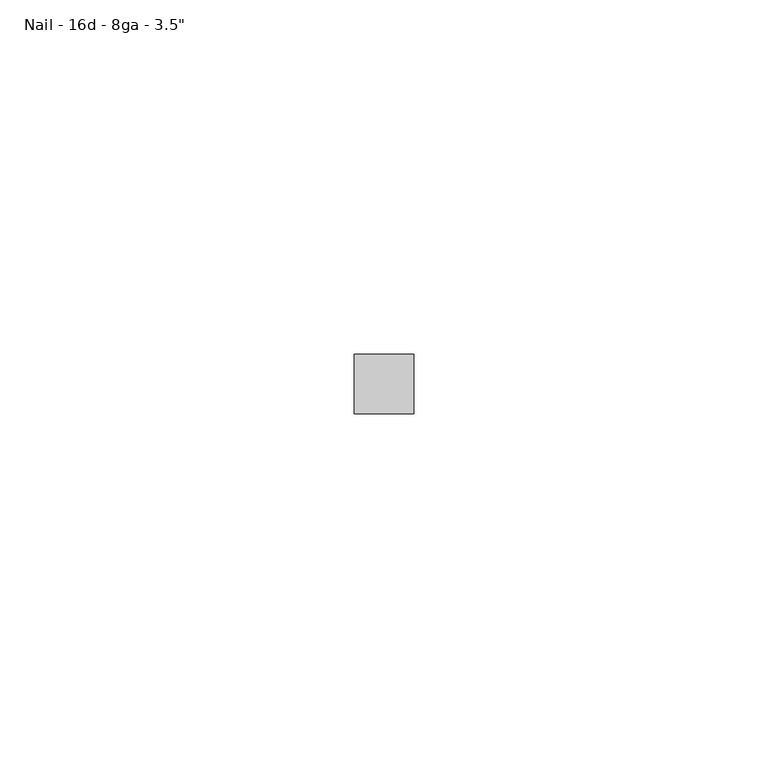
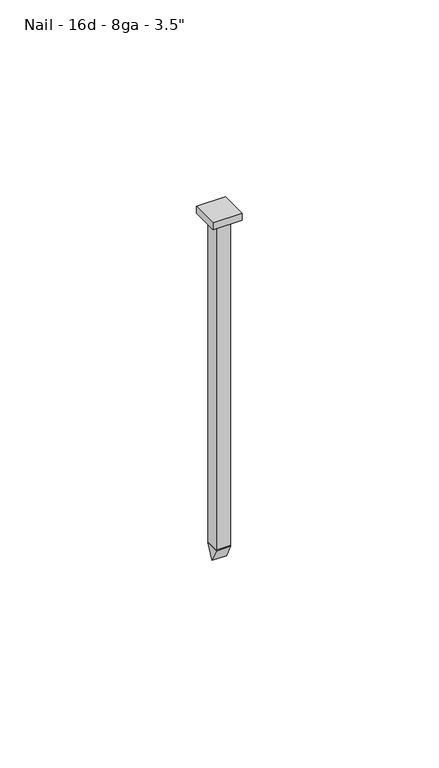
"""IFC4 building model written with IfcOpenShell, lengths in millimetres: fastener geometry."""

from ifc_helpers import new_model, si_unit, frame, origin, origin_with_axes, place, context, project, spatial, polyline, outline, extrude, source, transform, mapped, element, save


def fastener_034bf7df(model_context):
    return source(origin(), model_context, "Body", "SweptSolid", [
        extrude(outline(polyline([(0.0, -105.791), (-2.0955, -101.6), (2.0955, -101.6), (0.0, -105.791)])), frame((-2.0955, 0.0, 0.0), z_axis=(1.0, 0.0, 0.0), x_axis=(0.0, 1.0, 0.0)), (0.0, 0.0, 1.0), 4.191),
        extrude(outline(polyline([(-4.191, -4.191), (-4.191, 4.191), (4.191, 4.191), (4.191, -4.191), (-4.191, -4.191)])), origin_with_axes(), (0.0, 0.0, 1.0), 2.0955),
        extrude(outline(polyline([(-2.0955, 2.0955), (2.0955, 2.0955), (2.0955, -2.0955), (-2.0955, -2.0955), (-2.0955, 2.0955)])), frame((0.0, 0.0, -101.6), z_axis=(0.0, 0.0, 1.0), x_axis=(1.0, 0.0, 0.0)), (0.0, 0.0, 1.0), 101.6),
    ])


if __name__ == "__main__":
    model = new_model("IFC4")
    model_context = context("Model", 3, world=origin())
    ifc_project = project(units=[si_unit("LENGTHUNIT", "METRE", prefix="MILLI")], contexts=[model_context])
    site = spatial("IfcSite", under=ifc_project)
    building = spatial("IfcBuilding", under=site)
    placement = place(None, origin())
    fastener_shape = fastener_034bf7df(model_context)
    element("IfcFastener", 1, ObjectType="060523 - W_P_C - Fastenings - Generic - SQUARE : Nail - 16d - 8ga - 3.5\"", at=placement, inside=building, context=model_context, shape_type="MappedRepresentation", body=[
        mapped(fastener_shape, transform((0.0, 0.0, 0.0), x_axis=(1.0, 0.0, 0.0), y_axis=(0.0, 1.0, 0.0), z_axis=(0.0, 0.0, 1.0))),
    ])
    save(model, "model.ifc")

# Revit data of these elements
# Project information
#   Project Issue Date = "Issue Date"
#   Project Status = "Project Status"
#   Client Name = "Owner"
#   Project Address = "Enter address here"
#   Project Name = "Project Name"
#   Project Number = "Project Number"
# Type "060523 - W_P_C - Fastenings - Generic - SQUARE : Nail - 16d - 8ga - 3.5\""
#   Washer_Thickness = 0' - 0.00333"
#   Washer Radius = 0' - 0.0925"
#   Washer Offset - Head = 0' - 0"
#   Washer Offset = 0' - 0"
#   Thickness_of_Substrate [instance default] = 0' - 1"
#   Side = 0' - 0 37/64"
#   Radius = 0' - 0.0825"
#   Length [instance default] = 0' - 3 1/2"
#   Head Size = 0' - 1"
#   Head Radius = 0' - 0 1/2"
#   Head Height = 0' - 0.01"
#   Double Diameter = 0' - 0.33"
#   Diameter = 0' - 0.165"
#   Default Elevation = 4' - 0"
#   Washer_Nut_Visibility = no
#   Washer_Head_Visibility = no
#   Round_Head_Visibility = yes
#   Point Visibility = yes
#   Nut_Visibility = no
#   Hex_Head_Visiblilty = no
#   Washer Material = none
#   Bolt Material (Size) = AT SILL - FASTENER AT 24" O.C.
# Element 1 (IfcFastener, "060523 - W_P_C - Fastenings - Generic - SQUARE : Nail - 16d - 8ga - 3.5\"")
#   Length = 0' - 4"
# Materials
#   "AT SILL - FASTENER AT 24\" O.C.": class "Generic", colour RGB 120 120 120, transparency 0, Cost = 0
